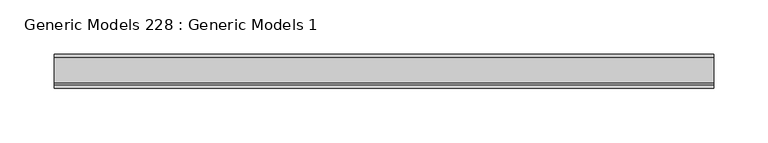
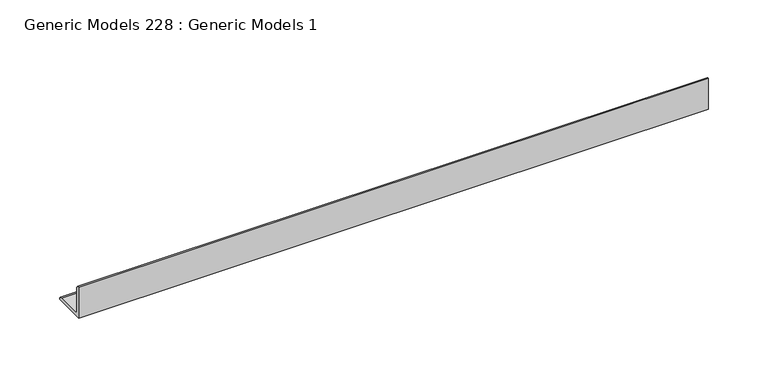
"""IFC4 building model written with IfcOpenShell, lengths in millimetres: proxy geometry, Generic Models 228 : Generic Models 1."""

from ifc_helpers import new_model, si_unit, point, frame, frame_2d, origin, place, context, project, spatial, polyline, circle_curve, trimmed, segment, composite_curve, outline, extrude, source, transform, mapped, element, save


def generic_models_228_generic_models_1_4406b45e(model_context):
    return source(origin(), model_context, "Body", "SweptSolid", [
        extrude(outline(composite_curve([segment(polyline([(592.1375, 2311.0026794), (592.1375, 2342.7526794)]), True, "CONTINUOUS"), segment(trimmed(circle_curve(frame_2d((592.1375, 2339.5776794)), 3.175), [point((592.1375, 2342.7526794))], [point((595.3125, 2339.5776794))], False, "CARTESIAN"), True, "CONTINUOUS"), segment(polyline([(595.3125, 2339.5776794), (595.3125, 2315.7651794)]), True, "CONTINUOUS"), segment(trimmed(circle_curve(frame_2d((596.9, 2315.7651794)), 1.5875), [point((595.3125, 2315.7651794))], [point((596.9, 2314.1776794))], True, "CARTESIAN"), True, "CONTINUOUS"), segment(polyline([(596.9, 2314.1776794), (620.7125, 2314.1776794)]), True, "CONTINUOUS"), segment(trimmed(circle_curve(frame_2d((620.7125, 2311.0026794)), 3.175), [point((620.7125, 2314.1776794))], [point((623.8875, 2311.0026794))], False, "CARTESIAN"), True, "CONTINUOUS"), segment(polyline([(623.8875, 2311.0026794), (592.1375, 2311.0026794)]), True, "CONTINUOUS")], self_intersect=False)), frame((49619.9071108, 0.0, 0.0), z_axis=(1.0, 0.0, 0.0), x_axis=(0.0, 1.0, 0.0)), (0.0, 0.0, 1.0), 609.6),
    ])


if __name__ == "__main__":
    model = new_model("IFC4")
    model_context = context("Model", 3, world=origin())
    ifc_project = project(units=[si_unit("LENGTHUNIT", "METRE", prefix="MILLI")], contexts=[model_context])
    site = spatial("IfcSite", under=ifc_project)
    building = spatial("IfcBuilding", under=site)
    placement = place(None, origin())
    generic_models_228_generic_models_1_shape = generic_models_228_generic_models_1_4406b45e(model_context)
    element("IfcBuildingElementProxy", 1, Name="Generic Models 228 : Generic Models 1", ObjectType="Generic Models 228 : Generic Models 1", at=placement, inside=building, context=model_context, shape_type="MappedRepresentation", body=[
        mapped(generic_models_228_generic_models_1_shape, transform((0.0, 0.0, 0.0), x_axis=(1.0, 0.0, 0.0), y_axis=(0.0, 1.0, 0.0), z_axis=(0.0, 0.0, 1.0))),
    ])
    save(model, "model.ifc")

# Revit data of these elements
# Element 1 (IfcBuildingElementProxy, "Generic Models 228 : Generic Models 1")
#   Materials on its faces: "BULKHEAD FRAME WORK"
# Materials
#   "BULKHEAD FRAME WORK": class "Metal", colour RGB 189 187 185, transparency 0, Description = "Structural steel 50ksi", Cost = 0
